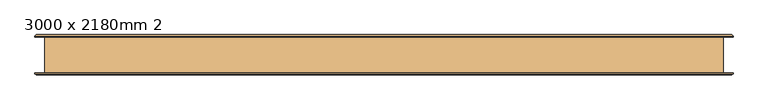
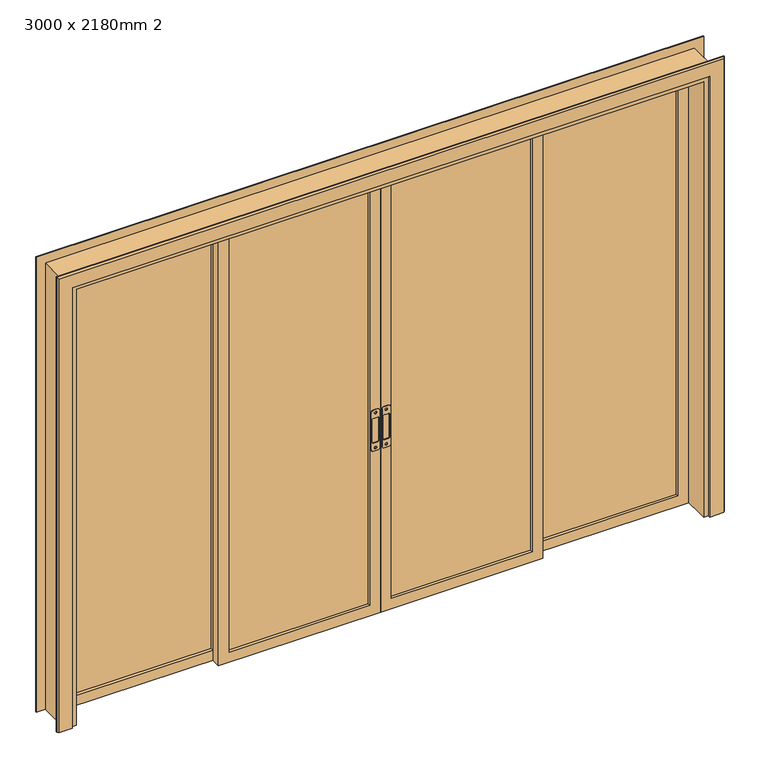
"""IFC4 building model written with IfcOpenShell, lengths in millimetres: door geometry, Porta envidraçada de correr quádrupla com revestimento : 3000 x 2180mm 2."""

from ifc_helpers import new_model, si_unit, point, frame, frame_2d, origin, place, context, project, spatial, polyline, circle_curve, trimmed, segment, composite_curve, outline, extrude, faceted_brep, source, transform, mapped, element, save


def door_3000_x_2180mm_2_d34f1594(model_context):
    return source(origin(), model_context, "Body", "SolidModel", [
        extrude(outline(composite_curve([segment(trimmed(circle_curve(frame_2d((990.0, 15.0)), 10.0), [point((1000.0, 15.0))], [point((990.0, 5.0))], False, "CARTESIAN"), True, "CONTINUOUS"), segment(polyline([(990.0, 5.0), (810.0, 5.0)]), True, "CONTINUOUS"), segment(trimmed(circle_curve(frame_2d((810.0, 15.0)), 10.0), [point((810.0, 5.0))], [point((800.0, 15.0))], False, "CARTESIAN"), True, "CONTINUOUS"), segment(polyline([(800.0, 15.0), (800.0, 35.0)]), True, "CONTINUOUS"), segment(trimmed(circle_curve(frame_2d((810.0, 35.0)), 10.0), [point((800.0, 35.0))], [point((810.0, 45.0))], False, "CARTESIAN"), True, "CONTINUOUS"), segment(polyline([(810.0, 45.0), (990.0, 45.0)]), True, "CONTINUOUS"), segment(trimmed(circle_curve(frame_2d((990.0, 35.0)), 10.0), [point((990.0, 45.0))], [point((1000.0, 35.0))], False, "CARTESIAN"), True, "CONTINUOUS"), segment(polyline([(1000.0, 35.0), (1000.0, 15.0)]), True, "CONTINUOUS")], self_intersect=False), holes=[composite_curve([segment(polyline([(960.0, 15.0), (960.0, 35.0)]), True, "CONTINUOUS"), segment(trimmed(circle_curve(frame_2d((955.0, 35.0)), 5.0), [point((960.0, 35.0))], [point((955.0, 40.0))], True, "CARTESIAN"), True, "CONTINUOUS"), segment(polyline([(955.0, 40.0), (845.0, 40.0)]), True, "CONTINUOUS"), segment(trimmed(circle_curve(frame_2d((845.0, 35.0)), 5.0), [point((845.0, 40.0))], [point((840.0, 35.0))], True, "CARTESIAN"), True, "CONTINUOUS"), segment(polyline([(840.0, 35.0), (840.0, 15.0)]), True, "CONTINUOUS"), segment(trimmed(circle_curve(frame_2d((845.0, 15.0)), 5.0), [point((840.0, 15.0))], [point((845.0, 10.0))], True, "CARTESIAN"), True, "CONTINUOUS"), segment(polyline([(845.0, 10.0), (955.0, 10.0)]), True, "CONTINUOUS"), segment(trimmed(circle_curve(frame_2d((955.0, 15.0)), 5.0), [point((955.0, 10.0))], [point((960.0, 15.0))], True, "CARTESIAN"), True, "CONTINUOUS")], self_intersect=False), composite_curve([segment(trimmed(circle_curve(frame_2d((985.0, 25.0)), 5.0), [point((985.0, 20.0))], [point((985.0, 30.0))], True, "CARTESIAN"), True, "CONTINUOUS"), segment(trimmed(circle_curve(frame_2d((985.0, 25.0)), 5.0), [point((985.0, 30.0))], [point((985.0, 20.0))], True, "CARTESIAN"), True, "CONTINUOUS")], self_intersect=False), composite_curve([segment(trimmed(circle_curve(frame_2d((815.0, 25.0)), 5.0), [point((815.0, 20.0))], [point((815.0, 30.0))], True, "CARTESIAN"), True, "CONTINUOUS"), segment(trimmed(circle_curve(frame_2d((815.0, 25.0)), 5.0), [point((815.0, 30.0))], [point((815.0, 20.0))], True, "CARTESIAN"), True, "CONTINUOUS")], self_intersect=False)]), frame((0.0, -8.4, 0.0), z_axis=(0.0, 1.0, 0.0), x_axis=(0.0, 0.0, 1.0)), (0.0, 0.0, 1.0), 3.0),
        extrude(outline(composite_curve([segment(trimmed(circle_curve(frame_2d((990.0, -35.0)), 10.0), [point((1000.0, -35.0))], [point((990.0, -45.0))], False, "CARTESIAN"), True, "CONTINUOUS"), segment(polyline([(990.0, -45.0), (810.0, -45.0)]), True, "CONTINUOUS"), segment(trimmed(circle_curve(frame_2d((810.0, -35.0)), 10.0), [point((810.0, -45.0))], [point((800.0, -35.0))], False, "CARTESIAN"), True, "CONTINUOUS"), segment(polyline([(800.0, -35.0), (800.0, -15.0)]), True, "CONTINUOUS"), segment(trimmed(circle_curve(frame_2d((810.0, -15.0)), 10.0), [point((800.0, -15.0))], [point((810.0, -5.0))], False, "CARTESIAN"), True, "CONTINUOUS"), segment(polyline([(810.0, -5.0), (990.0, -5.0)]), True, "CONTINUOUS"), segment(trimmed(circle_curve(frame_2d((990.0, -15.0)), 10.0), [point((990.0, -5.0))], [point((1000.0, -15.0))], False, "CARTESIAN"), True, "CONTINUOUS"), segment(polyline([(1000.0, -15.0), (1000.0, -35.0)]), True, "CONTINUOUS")], self_intersect=False), holes=[composite_curve([segment(polyline([(960.0, -35.0), (960.0, -15.0)]), True, "CONTINUOUS"), segment(trimmed(circle_curve(frame_2d((955.0, -15.0)), 5.0), [point((960.0, -15.0))], [point((955.0, -10.0))], True, "CARTESIAN"), True, "CONTINUOUS"), segment(polyline([(955.0, -10.0), (845.0, -10.0)]), True, "CONTINUOUS"), segment(trimmed(circle_curve(frame_2d((845.0, -15.0)), 5.0), [point((845.0, -10.0))], [point((840.0, -15.0))], True, "CARTESIAN"), True, "CONTINUOUS"), segment(polyline([(840.0, -15.0), (840.0, -35.0)]), True, "CONTINUOUS"), segment(trimmed(circle_curve(frame_2d((845.0, -35.0)), 5.0), [point((840.0, -35.0))], [point((845.0, -40.0))], True, "CARTESIAN"), True, "CONTINUOUS"), segment(polyline([(845.0, -40.0), (955.0, -40.0)]), True, "CONTINUOUS"), segment(trimmed(circle_curve(frame_2d((955.0, -35.0)), 5.0), [point((955.0, -40.0))], [point((960.0, -35.0))], True, "CARTESIAN"), True, "CONTINUOUS")], self_intersect=False), composite_curve([segment(trimmed(circle_curve(frame_2d((985.0, -25.0)), 5.0), [point((985.0, -30.0))], [point((985.0, -20.0))], True, "CARTESIAN"), True, "CONTINUOUS"), segment(trimmed(circle_curve(frame_2d((985.0, -25.0)), 5.0), [point((985.0, -20.0))], [point((985.0, -30.0))], True, "CARTESIAN"), True, "CONTINUOUS")], self_intersect=False), composite_curve([segment(trimmed(circle_curve(frame_2d((815.0, -25.0)), 5.0), [point((815.0, -30.0))], [point((815.0, -20.0))], True, "CARTESIAN"), True, "CONTINUOUS"), segment(trimmed(circle_curve(frame_2d((815.0, -25.0)), 5.0), [point((815.0, -20.0))], [point((815.0, -30.0))], True, "CARTESIAN"), True, "CONTINUOUS")], self_intersect=False)]), frame((0.0, -8.4, 0.0), z_axis=(0.0, 1.0, 0.0), x_axis=(0.0, 0.0, 1.0)), (0.0, 0.0, 1.0), 3.0),
        extrude(outline(polyline([(2130.0, 0.0), (2130.0, -750.0), (0.0, -750.0), (0.0, 0.0), (2130.0, 0.0)]), holes=[polyline([(2080.0, -700.0), (2080.0, -50.0), (50.0, -50.0), (50.0, -700.0), (2080.0, -700.0)])]), frame((0.0, -5.4, 0.0), z_axis=(0.0, 1.0, 0.0), x_axis=(0.0, 0.0, 1.0)), (0.0, 0.0, 1.0), 40.0),
        extrude(outline(polyline([(2130.0, 1450.0), (2130.0, 700.0), (0.0, 700.0), (0.0, 1450.0), (2130.0, 1450.0)]), holes=[polyline([(2080.0, 750.0), (2080.0, 1400.0), (50.0, 1400.0), (50.0, 750.0), (2080.0, 750.0)])]), frame((0.0, 39.6, 0.0), z_axis=(0.0, 1.0, 0.0), x_axis=(0.0, 0.0, 1.0)), (0.0, 0.0, 1.0), 40.0),
        extrude(outline(polyline([(2130.0, 750.0), (2130.0, 0.0), (0.0, 0.0), (0.0, 750.0), (2130.0, 750.0)]), holes=[polyline([(2080.0, 50.0), (2080.0, 700.0), (50.0, 700.0), (50.0, 50.0), (2080.0, 50.0)])]), frame((0.0, -5.4, 0.0), z_axis=(0.0, 1.0, 0.0), x_axis=(0.0, 0.0, 1.0)), (0.0, 0.0, 1.0), 40.0),
        extrude(outline(polyline([(2130.0, -700.0), (2130.0, -1450.0), (0.0, -1450.0), (0.0, -700.0), (2130.0, -700.0)]), holes=[polyline([(2080.0, -1400.0), (2080.0, -750.0), (50.0, -750.0), (50.0, -1400.0), (2080.0, -1400.0)])]), frame((0.0, 39.6, 0.0), z_axis=(0.0, 1.0, 0.0), x_axis=(0.0, 0.0, 1.0)), (0.0, 0.0, 1.0), 40.0),
        extrude(outline(polyline([(0.0, 1500.0), (2180.0, 1500.0), (2180.0, -1500.0), (0.0, -1500.0), (0.0, -1450.0), (2130.0, -1450.0), (2130.0, 1450.0), (0.0, 1450.0), (0.0, 1500.0)])), frame((0.0, -79.6, 0.0), z_axis=(0.0, 1.0, 0.0), x_axis=(0.0, 0.0, 1.0)), (0.0, 0.0, 1.0), 159.2),
        extrude(outline(polyline([(700.0, 7.6), (50.0, 7.6), (50.0, 21.6), (700.0, 21.6), (700.0, 7.6)])), frame((0.0, 0.0, 50.0), z_axis=(0.0, 0.0, 1.0), x_axis=(1.0, 0.0, 0.0)), (0.0, 0.0, 1.0), 2030.0),
        extrude(outline(polyline([(1400.0, 52.6), (750.0, 52.6), (750.0, 66.6), (1400.0, 66.6), (1400.0, 52.6)])), frame((0.0, 0.0, 50.0), z_axis=(0.0, 0.0, 1.0), x_axis=(1.0, 0.0, 0.0)), (0.0, 0.0, 1.0), 2030.0),
        extrude(outline(polyline([(-750.0, 52.6), (-1400.0, 52.6), (-1400.0, 66.6), (-750.0, 66.6), (-750.0, 52.6)])), frame((0.0, 0.0, 50.0), z_axis=(0.0, 0.0, 1.0), x_axis=(1.0, 0.0, 0.0)), (0.0, 0.0, 1.0), 2030.0),
        extrude(outline(polyline([(-50.0, 7.6), (-700.0, 7.6), (-700.0, 21.6), (-50.0, 21.6), (-50.0, 7.6)])), frame((0.0, 0.0, 50.0), z_axis=(0.0, 0.0, 1.0), x_axis=(1.0, 0.0, 0.0)), (0.0, 0.0, 1.0), 2030.0),
        extrude(outline(polyline([(-750.0, 52.6), (-1400.0, 52.6), (-1400.0, 66.6), (-750.0, 66.6), (-750.0, 52.6)])), frame((0.0, 0.0, 50.0), z_axis=(0.0, 0.0, 1.0), x_axis=(1.0, 0.0, 0.0)), (0.0, 0.0, 1.0), 2030.0),
        extrude(outline(polyline([(-50.0, 7.6), (-700.0, 7.6), (-700.0, 21.6), (-50.0, 21.6), (-50.0, 7.6)])), frame((0.0, 0.0, 50.0), z_axis=(0.0, 0.0, 1.0), x_axis=(1.0, 0.0, 0.0)), (0.0, 0.0, 1.0), 2030.0),
        extrude(outline(polyline([(750.0, 52.6), (750.0, 66.6), (1400.0, 66.6), (1400.0, 52.6), (750.0, 52.6)])), frame((0.0, 0.0, 50.0), z_axis=(0.0, 0.0, 1.0), x_axis=(1.0, 0.0, 0.0)), (0.0, 0.0, 1.0), 2030.0),
        extrude(outline(polyline([(50.0, 7.6), (50.0, 21.6), (700.0, 21.6), (700.0, 7.6), (50.0, 7.6)])), frame((0.0, 0.0, 50.0), z_axis=(0.0, 0.0, 1.0), x_axis=(1.0, 0.0, 0.0)), (0.0, 0.0, 1.0), 2030.0),
        faceted_brep([(1543.0, -83.6, 0.0), (1537.0, -89.6, 0.0), (1473.0, -89.6, 0.0), (1473.0, -79.6, 0.0), (1543.0, -79.6, 0.0), (1543.0, -79.6, 2223.0), (1543.0, -83.6, 2223.0), (1473.0, -79.6, 2153.0), (-1473.0, -79.6, 2153.0), (-1473.0, -79.6, 0.0), (-1543.0, -79.6, 0.0), (-1543.0, -79.6, 2223.0), (1473.0, -89.6, 2153.0), (1537.0, -89.6, 2217.0), (-1537.0, -89.6, 2217.0), (-1537.0, -89.6, 0.0), (-1473.0, -89.6, 0.0), (-1473.0, -89.6, 2153.0), (-1543.0, -83.6, 0.0), (-1543.0, -83.6, 2223.0)], [[[0, 1, 2, 3, 4]], [[4, 5, 6, 0]], [[3, 7, 8, 9, 10, 11, 5, 4]], [[2, 12, 7, 3]], [[1, 13, 14, 15, 16, 17, 12, 2]], [[0, 6, 13, 1]], [[17, 16, 9, 8]], [[18, 10, 9, 16, 15]], [[19, 18, 15, 14]], [[11, 10, 18, 19]], [[6, 19, 14, 13]], [[12, 17, 8, 7]], [[5, 11, 19, 6]]]),
        faceted_brep([(1543.0, 83.6, 0.0), (1543.0, 79.6, 0.0), (1473.0, 79.6, 0.0), (1473.0, 89.6, 0.0), (1537.0, 89.6, 0.0), (1537.0, 89.6, 2217.0), (1543.0, 83.6, 2223.0), (1473.0, 89.6, 2153.0), (-1473.0, 89.6, 2153.0), (-1473.0, 89.6, 0.0), (-1537.0, 89.6, 0.0), (-1537.0, 89.6, 2217.0), (1473.0, 79.6, 2153.0), (1543.0, 79.6, 2223.0), (-1543.0, 79.6, 2223.0), (-1543.0, 79.6, 0.0), (-1473.0, 79.6, 0.0), (-1473.0, 79.6, 2153.0), (-1543.0, 83.6, 0.0), (-1543.0, 83.6, 2223.0)], [[[0, 1, 2, 3, 4]], [[4, 5, 6, 0]], [[3, 7, 8, 9, 10, 11, 5, 4]], [[2, 12, 7, 3]], [[1, 13, 14, 15, 16, 17, 12, 2]], [[0, 6, 13, 1]], [[11, 10, 18, 19]], [[18, 10, 9, 16, 15]], [[17, 16, 9, 8]], [[19, 18, 15, 14]], [[5, 11, 19, 6]], [[12, 17, 8, 7]], [[6, 19, 14, 13]]]),
    ])


if __name__ == "__main__":
    model = new_model("IFC4")
    model_context = context("Model", 3, world=origin())
    ifc_project = project(units=[si_unit("LENGTHUNIT", "METRE", prefix="MILLI")], contexts=[model_context])
    site = spatial("IfcSite", under=ifc_project)
    building = spatial("IfcBuilding", under=site)
    placement = place(None, origin())
    door_3000_x_2180mm_2_shape = door_3000_x_2180mm_2_d34f1594(model_context)
    element("IfcDoor", 1, ObjectType="Porta envidraçada de correr quádrupla com revestimento : 3000 x 2180mm 2", at=placement, inside=building, context=model_context, shape_type="MappedRepresentation", body=[
        mapped(door_3000_x_2180mm_2_shape, transform((0.0, 0.0, 0.0), x_axis=(1.0, 0.0, 0.0), y_axis=(0.0, 1.0, 0.0), z_axis=(0.0, 0.0, 1.0))),
    ])
    save(model, "model.ifc")

# Revit data of these elements
# Type "Porta envidraçada de correr quádrupla com revestimento : 3000 x 2180mm 2"
#   Type Mark = "P32"
#   Construction Type Id = "GSP4R"
#   Analytic Construction = "Vidraça única Pilkington 1/8 pol"
#   Visual Light Transmittance = 0.9
#   Largura da apara = 0.07 m
#   Espessura da apara = 0.01 m
#   Solar Heat Gain Coefficient = 0.78
#   Rough Width = 3.00 m
#   Rough Height = 2.18 m
#   Largura da moldura do painel = 0.05 m
#   Espessura da moldura do painel = 0.04 m
#   Heat Transfer Coefficient (U) = 3.6886 W/(m²·K)
#   Largura da maçaneta = 0.04 m
#   Altura do puxador = 0.20 m
#   Largura da estrutura = 0.05 m
#   Height = 2.18 m
#   Width = 3.00 m
#   Function = 1
#   Material da apara = none
#   Material do puxador = none
#   Vidro = Vidro
#   Material da estrutura = none
#   Thickness = 0
#   Wall Closure = (empty or 0)
# Element 1 (IfcDoor, "Porta envidraçada de correr quádrupla com revestimento : 3000 x 2180mm 2")
#   Materials on its faces: "Vidro"
# Materials
#   "Vidro": class "Vidro", colour RGB 0 128 192, transparency 0.9, Description = "Vidro de sílica", Cost = 0
